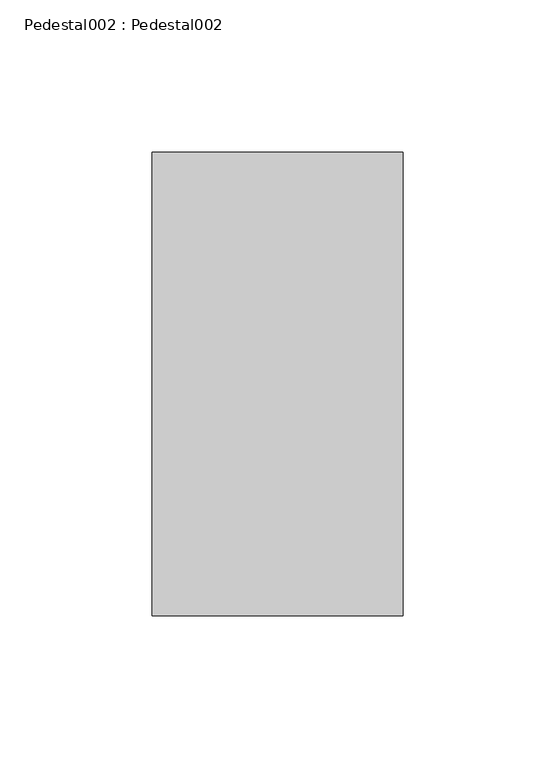
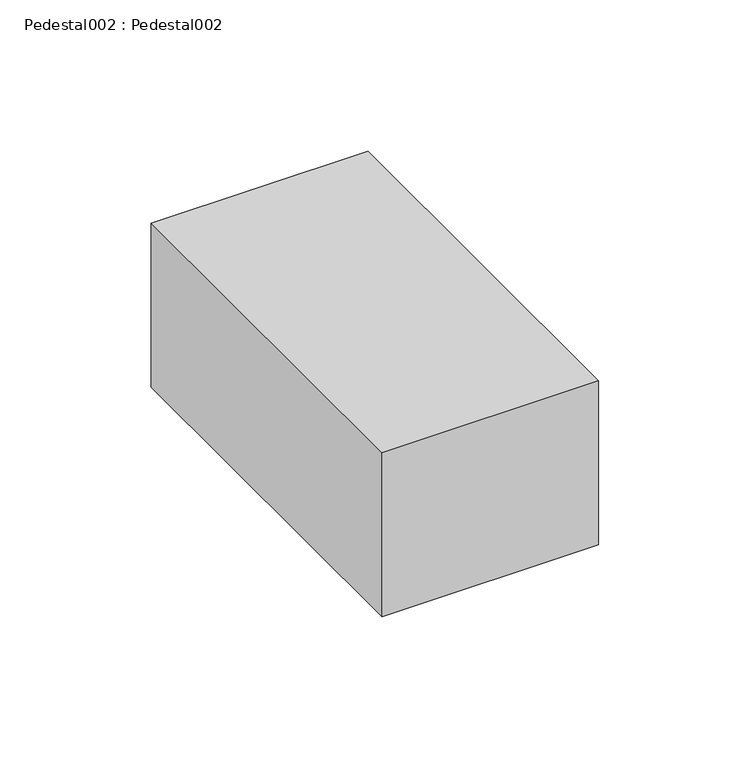
"""IFC4 building model written with IfcOpenShell, lengths in millimetres: proxy geometry, Pedestal002 : Pedestal002."""

from ifc_helpers import new_model, si_unit, frame, origin, place, context, project, spatial, polyline, outline, extrude, source, transform, mapped, element, save


def pedestal002_pedestal002_8a8a3094(model_context):
    return source(origin(), model_context, "Body", "SweptSolid", [
        extrude(outline(polyline([(-6928.6755859, 9829.7531721), (-7011.2255859, 9829.7531721), (-7011.2255859, 9982.1531721), (-6928.6755859, 9982.1531721), (-6928.6755859, 9829.7531721)])), frame((0.0, 0.0, 40124.2226562), z_axis=(0.0, 0.0, 1.0), x_axis=(1.0, 0.0, 0.0)), (0.0, 0.0, 1.0), 66.061023),
    ])


if __name__ == "__main__":
    model = new_model("IFC4")
    model_context = context("Model", 3, world=origin())
    ifc_project = project(units=[si_unit("LENGTHUNIT", "METRE", prefix="MILLI")], contexts=[model_context])
    site = spatial("IfcSite", under=ifc_project)
    building = spatial("IfcBuilding", under=site)
    placement = place(None, origin())
    pedestal002_pedestal002_shape = pedestal002_pedestal002_8a8a3094(model_context)
    element("IfcBuildingElementProxy", 1, Name="Pedestal002 : Pedestal002", ObjectType="Pedestal002 : Pedestal002", at=placement, inside=building, context=model_context, shape_type="MappedRepresentation", body=[
        mapped(pedestal002_pedestal002_shape, transform((0.0, 0.0, 0.0), x_axis=(1.0, 0.0, 0.0), y_axis=(0.0, 1.0, 0.0), z_axis=(0.0, 0.0, 1.0))),
    ])
    save(model, "model.ifc")

# Revit data of these elements
# Type "Pedestal002 : Pedestal002"
#   NameOverride = "Pedestal002"
# Element 1 (IfcBuildingElementProxy, "Pedestal002 : Pedestal002")
#   Materials on its faces: "BUZON PEDESTAL"
# Materials
#   "BUZON PEDESTAL": class "Unassigned", colour RGB 66 66 66, transparency 0
